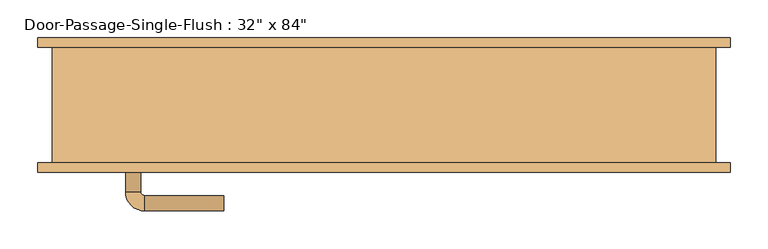
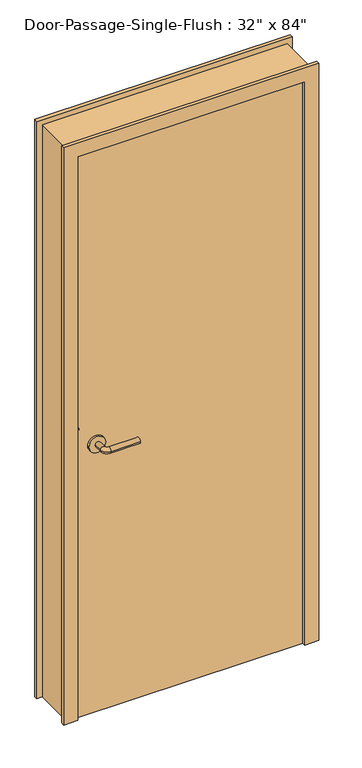
"""IFC4 building model written with IfcOpenShell, lengths in millimetres: door geometry."""

import ifcopenshell
import ifcopenshell.guid

model = None  # the IFC model being written
_history = None  # IfcOwnerHistory: only IFC2X3 demands one
_inside = {}  # id of a spatial element -> (the spatial element, [elements in it])
_under = {}  # id of a project, library or spatial element -> (it, [spatial elements below it])
_declared = {}  # id of a project -> (the project, [libraries it declares])
_typed = {}  # id of a type object -> (the type object, [elements of that type])
_made_of = {}  # id of a material, layer set ... -> (it, [elements and type objects made of it])


def new_model(schema):
    """Start an empty IFC model of exactly this schema.

    Asked for "IFC4X3", IfcOpenShell would pick the latest addendum, in which some entities
    have other attributes; the version numbers below select the first issue.
    IFC2X3 requires an IfcOwnerHistory on every rooted entity: one is made here for all.
    """
    global model, _history
    if schema == "IFC4X3":
        model = ifcopenshell.file(schema_version=(4, 3, 0, 0))
    else:
        model = ifcopenshell.file(schema=schema)
    _inside.clear()
    _under.clear()
    _declared.clear()
    _typed.clear()
    _made_of.clear()
    _history = None
    if model.schema == "IFC2X3":
        org = make("IfcOrganization", Name="unknown")
        user = make(
            "IfcPersonAndOrganization",
            ThePerson=make("IfcPerson", FamilyName="unknown"),
            TheOrganization=org,
        )
        app = make(
            "IfcApplication",
            ApplicationDeveloper=org,
            Version="unknown",
            ApplicationFullName="unknown",
            ApplicationIdentifier="unknown",
        )
        _history = make(
            "IfcOwnerHistory",
            OwningUser=user,
            OwningApplication=app,
            ChangeAction="ADDED",
            CreationDate=0,
        )
    return model


def make(cls, **values):
    """One entity of the class cls with the attributes given. An attribute that is None is left unset."""
    return model.create_entity(
        cls, **{name: value for name, value in values.items() if value is not None}
    )


def rooted(cls, **values):
    """An entity with a GlobalId (a new one), such as an element, a storey or a relation."""
    return make(cls, GlobalId=ifcopenshell.guid.new(), OwnerHistory=_history, **values)


def si_unit(unit_type, name, prefix=None):
    """IfcSIUnit, for example si_unit("LENGTHUNIT", "METRE", prefix="MILLI")."""
    return make("IfcSIUnit", UnitType=unit_type, Prefix=prefix, Name=name)


def assignment(units):
    """IfcUnitAssignment: the units of a project."""
    return None if units is None else make("IfcUnitAssignment", Units=units)


def point(xyz):
    """IfcCartesianPoint."""
    return None if xyz is None else make("IfcCartesianPoint", Coordinates=xyz)


def direction(xyz):
    """IfcDirection."""
    return None if xyz is None else make("IfcDirection", DirectionRatios=xyz)


def frame(location, z_axis=None, x_axis=None):
    """IfcAxis2Placement3D, a coordinate frame: its origin and axes. An axis left out is left unset."""
    return make(
        "IfcAxis2Placement3D",
        Location=point(location),
        Axis=direction(z_axis),
        RefDirection=direction(x_axis),
    )


def frame_2d(location, x_axis=None):
    """IfcAxis2Placement2D, a coordinate frame in the plane: its origin and x axis."""
    return make(
        "IfcAxis2Placement2D", Location=point(location), RefDirection=direction(x_axis)
    )


def origin():
    """The frame at (0, 0, 0) with its axes left unset."""
    return frame((0.0, 0.0, 0.0))


def origin_with_axes():
    """The frame at (0, 0, 0) with the z axis (0, 0, 1) and the x axis (1, 0, 0) written out."""
    return frame((0.0, 0.0, 0.0), z_axis=(0.0, 0.0, 1.0), x_axis=(1.0, 0.0, 0.0))


def place(relative_to, where):
    """IfcLocalPlacement: puts the frame where relative to a parent placement (None: the world)."""
    return make(
        "IfcLocalPlacement", PlacementRelTo=relative_to, RelativePlacement=where
    )


def context(
    kind, dimensions, precision=None, world=None, true_north=None, identifier=None
):
    """IfcGeometricRepresentationContext, for example the 3D "Model" context."""
    return make(
        "IfcGeometricRepresentationContext",
        ContextIdentifier=identifier,
        ContextType=kind,
        CoordinateSpaceDimension=dimensions,
        Precision=precision,
        WorldCoordinateSystem=world,
        TrueNorth=true_north,
    )


def project(units=None, contexts=None):
    """IfcProject with its units and contexts."""
    return rooted(
        "IfcProject",
        Name="project",
        RepresentationContexts=contexts,
        UnitsInContext=assignment(units),
    )


def spatial(cls, under=None, at=None, **own):
    """A site, building, storey or space (cls), placed at a placement, below another one or the project."""
    s = rooted(cls, ObjectPlacement=at, **own)
    if under is not None:
        _under.setdefault(under.id(), (under, []))[1].append(s)
    return s


def polyline(points):
    """IfcPolyline through the points."""
    return make("IfcPolyline", Points=[point(p) for p in points])


def circle_curve(where, radius):
    """IfcCircle in the frame where."""
    return make("IfcCircle", Position=where, Radius=radius)


def ellipse_curve(where, semi_axis1, semi_axis2):
    """IfcEllipse in the frame where."""
    return make(
        "IfcEllipse", Position=where, SemiAxis1=semi_axis1, SemiAxis2=semi_axis2
    )


def trimmed(basis, trim1, trim2, sense, master):
    """IfcTrimmedCurve: the piece of a basis curve between two trims."""
    return make(
        "IfcTrimmedCurve",
        BasisCurve=basis,
        Trim1=trim1,
        Trim2=trim2,
        SenseAgreement=sense,
        MasterRepresentation=master,
    )


def segment(curve, same_sense, transition):
    """IfcCompositeCurveSegment."""
    return make(
        "IfcCompositeCurveSegment",
        Transition=transition,
        SameSense=same_sense,
        ParentCurve=curve,
    )


def composite_curve(segments, self_intersect=None):
    """IfcCompositeCurve: segments joined end to end."""
    return make("IfcCompositeCurve", Segments=segments, SelfIntersect=self_intersect)


def outline(outer, holes=None, kind="AREA"):
    """IfcArbitraryClosedProfileDef: a profile drawn as a closed curve; with holes, ...WithVoids."""
    if holes is None:
        return make("IfcArbitraryClosedProfileDef", ProfileType=kind, OuterCurve=outer)
    return make(
        "IfcArbitraryProfileDefWithVoids",
        ProfileType=kind,
        OuterCurve=outer,
        InnerCurves=holes,
    )


def extrude(swept, where, along, depth):
    """IfcExtrudedAreaSolid: the profile swept, set in the frame where, extruded along a direction by depth."""
    return make(
        "IfcExtrudedAreaSolid",
        SweptArea=swept,
        Position=where,
        ExtrudedDirection=direction(along),
        Depth=depth,
    )


def faces_of(points, faces, orient=None, outer=None):
    """IfcFace entities. A face is a list of loops; a loop is a list of indices into points, from 0.

    orient and outer hold one flag for each loop. By default every Orientation is true, the
    first loop of a face is its IfcFaceOuterBound and the others are IfcFaceBound.
    """
    made = []
    for i, loops in enumerate(faces):
        bounds = []
        for j, loop in enumerate(loops):
            is_outer = j == 0 if outer is None else outer[i][j]
            bounds.append(
                make(
                    "IfcFaceOuterBound" if is_outer else "IfcFaceBound",
                    Bound=make("IfcPolyLoop", Polygon=[points[k] for k in loop]),
                    Orientation=True if orient is None else orient[i][j],
                )
            )
        made.append(make("IfcFace", Bounds=bounds))
    return made


def faceted_brep(points, faces, orient=None, outer=None, voids=None):
    """IfcFacetedBrep: a solid bounded by flat faces; with voids (closed shells), ...WithVoids."""
    shared = [point(p) for p in points]
    hull = make("IfcClosedShell", CfsFaces=faces_of(shared, faces, orient, outer))
    if voids is None:
        return make("IfcFacetedBrep", Outer=hull)
    return make(
        "IfcFacetedBrepWithVoids",
        Outer=hull,
        Voids=[
            make(cls, CfsFaces=faces_of(shared, fs, o, b)) for cls, fs, o, b in voids
        ],
    )


def shape(context_of_items, identifier, shape_type, items):
    """IfcShapeRepresentation: the items that make up one representation, for example the "Body"."""
    return make(
        "IfcShapeRepresentation",
        ContextOfItems=context_of_items,
        RepresentationIdentifier=identifier,
        RepresentationType=shape_type,
        Items=items,
    )


def source(mapping_origin, context_of_items, identifier, shape_type, items):
    """IfcRepresentationMap: a shape defined once, which mapped items show again and again."""
    return make(
        "IfcRepresentationMap",
        MappingOrigin=mapping_origin,
        MappedRepresentation=shape(context_of_items, identifier, shape_type, items),
    )


def transform(
    local_origin,
    x_axis=None,
    y_axis=None,
    z_axis=None,
    scale=None,
    scale2=None,
    scale3=None,
    uniform=True,
):
    """IfcCartesianTransformationOperator3D, or its non-uniform kind. x_axis, y_axis, z_axis: its Axis1, 2, 3."""
    if uniform:
        return make(
            "IfcCartesianTransformationOperator3D",
            Axis1=direction(x_axis),
            Axis2=direction(y_axis),
            LocalOrigin=point(local_origin),
            Scale=scale,
            Axis3=direction(z_axis),
        )
    return make(
        "IfcCartesianTransformationOperator3DnonUniform",
        Axis1=direction(x_axis),
        Axis2=direction(y_axis),
        LocalOrigin=point(local_origin),
        Scale=scale,
        Axis3=direction(z_axis),
        Scale2=scale2,
        Scale3=scale3,
    )


def mapped(mapping_source, mapping_target):
    """IfcMappedItem: shows the shape of a source again, moved by a transform."""
    return make(
        "IfcMappedItem", MappingSource=mapping_source, MappingTarget=mapping_target
    )


def made_of(thing, what):
    """Note that an element or type object is made of a material, layer set ...; save() writes the relation."""
    if what is not None:
        _made_of.setdefault(what.id(), (what, []))[1].append(thing)
    return thing


def element(
    cls,
    number,
    at=None,
    inside=None,
    cuts=None,
    type_object=None,
    material=None,
    context=None,
    identifier="Body",
    shape_type=None,
    held_by="IfcProductDefinitionShape",
    body=None,
    shapes=None,
    **own,
):
    """One element of the class cls, such as IfcWall. Its Tag is "e" and its number.

    at: its placement. inside: the storey or other place that contains it. cuts: it is an
    opening in that element (IfcRelVoidsElement). A single representation is given by context,
    identifier, shape_type and body (its items); several are given by shapes. held_by: the class
    of the entity that holds the representations. save() writes the other relations.
    """
    e = rooted(cls, Tag="e%d" % number, ObjectPlacement=at, **own)
    if body is not None:
        shapes = [shape(context, identifier, shape_type, body)]
    if shapes is not None:
        e.Representation = make(held_by, Representations=shapes)
    if inside is not None:
        _inside.setdefault(inside.id(), (inside, []))[1].append(e)
    if cuts is not None:
        rooted(
            "IfcRelVoidsElement", RelatingBuildingElement=cuts, RelatedOpeningElement=e
        )
    if type_object is not None:
        _typed.setdefault(type_object.id(), (type_object, []))[1].append(e)
    return made_of(e, material)


def aggregate(whole, parts):
    """IfcRelAggregates: a whole, such as a stair, and the parts it consists of."""
    return rooted("IfcRelAggregates", RelatingObject=whole, RelatedObjects=parts)


def save(model, path):
    """Write the relations noted so far, then the file.

    IfcRelAggregates (storeys below a building ...), IfcRelContainedInSpatialStructure (elements
    in a storey), IfcRelDefinesByType, IfcRelAssociatesMaterial and IfcRelDeclares: one each for
    every whole, place, type object, material and project.
    """
    for whole, parts in _under.values():
        aggregate(whole, parts)
    for where, things in _inside.values():
        rooted(
            "IfcRelContainedInSpatialStructure",
            RelatedElements=things,
            RelatingStructure=where,
        )
    for kind, things in _typed.values():
        rooted("IfcRelDefinesByType", RelatedObjects=things, RelatingType=kind)
    for what, things in _made_of.values():
        rooted("IfcRelAssociatesMaterial", RelatedObjects=things, RelatingMaterial=what)
    for by, libraries in _declared.values():
        rooted("IfcRelDeclares", RelatingContext=by, RelatedDefinitions=libraries)
    model.write(path)


def plane_surface(at):
    """IfcPlane: the flat surface through the origin of the frame at, square to its z axis."""
    return make("IfcPlane", Position=at)


def cylinder_surface(at, radius):
    """IfcCylindricalSurface: all points at the distance radius from the z axis of the frame at."""
    return make("IfcCylindricalSurface", Position=at, Radius=radius)


def revolved_surface(curve, axis_point, axis_direction):
    """IfcSurfaceOfRevolution: the curve turned about the line through axis_point along axis_direction."""
    return make(
        "IfcSurfaceOfRevolution",
        SweptCurve=make("IfcArbitraryOpenProfileDef", ProfileType="CURVE", Curve=curve),
        AxisPosition=make("IfcAxis1Placement", Location=point(axis_point), Axis=direction(axis_direction)),
    )


def advanced_brep(points, edges, surfaces, faces):
    """IfcAdvancedBrep: a solid bounded by faces that lie on surfaces and meet in shared edges.

    An edge is (start, end): straight between two places in points (the first is 0);
    or (start, end, curve); or (start, end, curve, False) where it runs against its curve.
    A face is (place in surfaces, loops), or (place, loops, False) where it looks against
    its surface's normal. A loop lists edges by number (the first is 1), with a minus sign
    where the edge is run from its end to its start. The first loop is the outer one.
    """
    corners = [point(p) for p in points]
    vertices = [make("IfcVertexPoint", VertexGeometry=c) for c in corners]
    made = []
    for start, end, *more in edges:
        made.append(
            make(
                "IfcEdgeCurve",
                EdgeStart=vertices[start],
                EdgeEnd=vertices[end],
                EdgeGeometry=more[0] if more else make("IfcPolyline", Points=[corners[start], corners[end]]),
                SameSense=more[1] if len(more) > 1 else True,
            )
        )
    hull = []
    for where, loops, *sense in faces:
        bounds = []
        for j, loop in enumerate(loops):
            ring = [make("IfcOrientedEdge", EdgeElement=made[abs(k) - 1], Orientation=k > 0) for k in loop]
            bounds.append(
                make(
                    "IfcFaceOuterBound" if j == 0 else "IfcFaceBound",
                    Bound=make("IfcEdgeLoop", EdgeList=ring),
                    Orientation=True,
                )
            )
        hull.append(make("IfcAdvancedFace", Bounds=bounds, FaceSurface=surfaces[where], SameSense=sense[0] if sense else True))
    return make("IfcAdvancedBrep", Outer=make("IfcClosedShell", CfsFaces=hull))


def door_3d684360(model_context):
    return source(origin(), model_context, "Body", "SolidModel", [
        advanced_brep(
        [(-341.390625, -23.75, 1016.0), (-321.390625, -23.75, 1016.0), (-341.390625, 6.25, 1016.0), (-321.390625, 6.25, 1016.0), (-316.390625, 11.25, 1016.0), (-316.390625, 31.25, 1016.0), (-211.390625, 31.25, 1016.0), (-211.390625, 11.25, 1016.0)],
        [
            (0, 1, circle_curve(frame((-331.390625, -23.75, 1016.0), z_axis=(0.0, -1.0, 0.0), x_axis=(1.0, 0.0, 0.0)), 10.0)),
            (1, 0, circle_curve(frame((-331.390625, -23.75, 1016.0), z_axis=(0.0, -1.0, 0.0), x_axis=(1.0, 0.0, 0.0)), 10.0)),
            (0, 2),
            (2, 3, circle_curve(frame((-331.390625, 6.25, 1016.0), z_axis=(0.0, -1.0, 0.0), x_axis=(1.0, 0.0, 0.0)), 10.0)),
            (3, 1),
            (3, 2, circle_curve(frame((-331.390625, 6.25, 1016.0), z_axis=(0.0, -1.0, 0.0), x_axis=(1.0, 0.0, 0.0)), 10.0)),
            (4, 3, circle_curve(frame((-316.390625, 6.25, 1016.0), z_axis=(0.0, 0.0, 1.0), x_axis=(-1.0, 0.0, 0.0)), 5.0)),
            (2, 5, circle_curve(frame((-316.390625, 6.25, 1016.0), z_axis=(0.0, 0.0, -1.0), x_axis=(-1.0, 0.0, 0.0)), 25.0)),
            (5, 4, circle_curve(frame((-316.390625, 21.25, 1016.0), z_axis=(-1.0, 0.0, 0.0), x_axis=(0.0, -1.0, 0.0)), 10.0)),
            (4, 5, circle_curve(frame((-316.390625, 21.25, 1016.0), z_axis=(-1.0, 0.0, 0.0), x_axis=(0.0, -1.0, 0.0)), 10.0)),
            (6, 7, circle_curve(frame((-211.390625, 21.25, 1016.0), z_axis=(1.0, 0.0, 0.0), x_axis=(0.0, -1.0, 0.0)), 10.0)),
            (7, 6, circle_curve(frame((-211.390625, 21.25, 1016.0), z_axis=(1.0, 0.0, 0.0), x_axis=(0.0, -1.0, 0.0)), 10.0)),
            (5, 6),
            (7, 4),
        ],
        [
            plane_surface(frame((-331.390625, -23.75, 1016.0), z_axis=(0.0, -1.0, 0.0), x_axis=(0.0, 0.0, 1.0))),
            cylinder_surface(frame((-331.390625, -23.75, 1016.0), z_axis=(0.0, -1.0, 0.0), x_axis=(1.0, 0.0, 0.0)), 10.0),
            revolved_surface(trimmed(ellipse_curve(frame((-331.390625, 6.25, 1016.0), z_axis=(0.0, -1.0, 0.0), x_axis=(1.0, 0.0, 0.0)), 10.0, 10.0), [point((-341.390625, 6.25, 1016.0))], [point((-321.390625, 6.25, 1016.0))], True, "CARTESIAN"), (-316.390625, 6.25, 1016.0), (0.0, 0.0, -1.0)),
            revolved_surface(trimmed(ellipse_curve(frame((-331.390625, 6.25, 1016.0), z_axis=(0.0, -1.0, 0.0), x_axis=(1.0, 0.0, 0.0)), 10.0, 10.0), [point((-321.390625, 6.25, 1016.0))], [point((-341.390625, 6.25, 1016.0))], True, "CARTESIAN"), (-316.390625, 6.25, 1016.0), (0.0, 0.0, -1.0)),
            plane_surface(frame((-211.390625, 21.25, 1016.0), z_axis=(1.0, 0.0, 0.0), x_axis=(0.0, 0.0, 1.0))),
            cylinder_surface(frame((-316.390625, 21.25, 1016.0), z_axis=(-1.0, 0.0, 0.0), x_axis=(0.0, -1.0, 0.0)), 10.0),
        ],
        [
            (0, [[1, 2]]),
            (1, [[-1, 3, 4, 5]]),
            (1, [[-2, -5, 6, -3]]),
            (2, [[7, -4, 8, 9]]),
            (3, [[-8, -6, -7, 10]]),
            (4, [[11, 12]]),
            (5, [[-9, 13, -12, 14]]),
            (5, [[-10, -14, -11, -13]]),
        ],
    ),
        extrude(outline(composite_curve([segment(trimmed(circle_curve(frame_2d((1016.0, -333.890625)), 30.0), [point((1016.0, -363.890625))], [point((1016.0, -303.890625))], False, "CARTESIAN"), True, "CONTINUOUS"), segment(trimmed(circle_curve(frame_2d((1016.0, -333.890625)), 30.0), [point((1016.0, -303.890625))], [point((1016.0, -363.890625))], False, "CARTESIAN"), True, "CONTINUOUS")], self_intersect=False)), frame((0.0, -31.75, 0.0), z_axis=(0.0, 1.0, 0.0), x_axis=(0.0, 0.0, 1.0)), (0.0, 0.0, 1.0), 8.0),
        advanced_brep(
        [(-341.390625, -90.55, 1016.0), (-321.390625, -90.55, 1016.0), (-321.390625, -120.55, 1016.0), (-341.390625, -120.55, 1016.0), (-316.390625, -125.55, 1016.0), (-316.390625, -145.55, 1016.0), (-211.390625, -145.55, 1016.0), (-211.390625, -125.55, 1016.0)],
        [
            (0, 1, circle_curve(frame((-331.390625, -90.55, 1016.0), z_axis=(0.0, 1.0, 0.0), x_axis=(1.0, 0.0, 0.0)), 10.0)),
            (1, 0, circle_curve(frame((-331.390625, -90.55, 1016.0), z_axis=(0.0, 1.0, 0.0), x_axis=(1.0, 0.0, 0.0)), 10.0)),
            (1, 2),
            (2, 3, circle_curve(frame((-331.390625, -120.55, 1016.0), z_axis=(0.0, 1.0, 0.0), x_axis=(1.0, 0.0, 0.0)), 10.0)),
            (3, 0),
            (3, 2, circle_curve(frame((-331.390625, -120.55, 1016.0), z_axis=(0.0, 1.0, 0.0), x_axis=(1.0, 0.0, 0.0)), 10.0)),
            (4, 5, circle_curve(frame((-316.390625, -135.55, 1016.0), z_axis=(-1.0, 0.0, 0.0), x_axis=(0.0, 1.0, 0.0)), 10.0)),
            (5, 3, circle_curve(frame((-316.390625, -120.55, 1016.0), z_axis=(0.0, 0.0, -1.0), x_axis=(-1.0, 0.0, 0.0)), 25.0)),
            (2, 4, circle_curve(frame((-316.390625, -120.55, 1016.0), z_axis=(0.0, 0.0, 1.0), x_axis=(-1.0, 0.0, 0.0)), 5.0)),
            (5, 4, circle_curve(frame((-316.390625, -135.55, 1016.0), z_axis=(-1.0, 0.0, 0.0), x_axis=(0.0, 1.0, 0.0)), 10.0)),
            (6, 7, circle_curve(frame((-211.390625, -135.55, 1016.0), z_axis=(1.0, 0.0, 0.0), x_axis=(0.0, 1.0, 0.0)), 10.0)),
            (7, 6, circle_curve(frame((-211.390625, -135.55, 1016.0), z_axis=(1.0, 0.0, 0.0), x_axis=(0.0, 1.0, 0.0)), 10.0)),
            (4, 7),
            (6, 5),
        ],
        [
            plane_surface(frame((-331.390625, -90.55, 1016.0), z_axis=(0.0, 1.0, 0.0), x_axis=(0.0, 0.0, 1.0))),
            cylinder_surface(frame((-331.390625, -90.55, 1016.0), z_axis=(0.0, 1.0, 0.0), x_axis=(1.0, 0.0, 0.0)), 10.0),
            revolved_surface(trimmed(ellipse_curve(frame((-331.390625, -120.55, 1016.0), z_axis=(0.0, -1.0, 0.0), x_axis=(1.0, 0.0, 0.0)), 10.0, 10.0), [point((-341.390625, -120.55, 1016.0))], [point((-321.390625, -120.55, 1016.0))], True, "CARTESIAN"), (-316.390625, -120.55, 1016.0), (0.0, 0.0, -1.0)),
            revolved_surface(trimmed(ellipse_curve(frame((-331.390625, -120.55, 1016.0), z_axis=(0.0, -1.0, 0.0), x_axis=(1.0, 0.0, 0.0)), 10.0, 10.0), [point((-321.390625, -120.55, 1016.0))], [point((-341.390625, -120.55, 1016.0))], True, "CARTESIAN"), (-316.390625, -120.55, 1016.0), (0.0, 0.0, -1.0)),
            plane_surface(frame((-211.390625, -135.55, 1016.0), z_axis=(1.0, 0.0, 0.0), x_axis=(0.0, 0.0, 1.0))),
            cylinder_surface(frame((-316.390625, -135.55, 1016.0), z_axis=(-1.0, 0.0, 0.0), x_axis=(0.0, 1.0, 0.0)), 10.0),
        ],
        [
            (0, [[1, 2]]),
            (1, [[3, 4, 5, -2]]),
            (1, [[-5, 6, -3, -1]]),
            (2, [[7, 8, -4, 9]]),
            (3, [[10, -9, -6, -8]]),
            (4, [[11, 12]]),
            (5, [[13, -11, 14, -7]]),
            (5, [[-14, -12, -13, -10]]),
        ],
    ),
        extrude(outline(composite_curve([segment(trimmed(circle_curve(frame_2d((1016.0, -333.890625)), 30.0), [point((1016.0, -363.890625))], [point((1016.0, -303.890625))], False, "CARTESIAN"), True, "CONTINUOUS"), segment(trimmed(circle_curve(frame_2d((1016.0, -333.890625)), 30.0), [point((1016.0, -303.890625))], [point((1016.0, -363.890625))], False, "CARTESIAN"), True, "CONTINUOUS")], self_intersect=False)), frame((0.0, -90.55, 0.0), z_axis=(0.0, 1.0, 0.0), x_axis=(0.0, 0.0, 1.0)), (0.0, 0.0, 1.0), 8.0),
        faceted_brep([(406.4, -95.25, 0.0), (406.4, -26.9875, 0.0), (390.525, -26.9875, 0.0), (390.525, 11.1125, 0.0), (406.4, 11.1125, 0.0), (406.4, 82.55, 0.0), (457.2, 82.55, 0.0), (457.2, 69.85, 0.0), (438.15, 69.85, 0.0), (438.15, -82.55, 0.0), (457.2, -82.55, 0.0), (457.2, -95.25, 0.0), (457.2, -95.25, 2184.4), (-457.2, -95.25, 2184.4), (-457.2, -95.25, 0.0), (-406.4, -95.25, 0.0), (-406.4, -95.25, 2133.6), (406.4, -95.25, 2133.6), (457.2, -82.55, 2184.4), (438.15, -82.55, 2165.35), (-438.15, -82.55, 2165.35), (-438.15, -82.55, 0.0), (-457.2, -82.55, 0.0), (-457.2, -82.55, 2184.4), (438.15, 69.85, 2165.35), (457.2, 69.85, 2184.4), (-457.2, 69.85, 2184.4), (-457.2, 69.85, 0.0), (-438.15, 69.85, 0.0), (-438.15, 69.85, 2165.35), (457.2, 82.55, 2184.4), (406.4, 82.55, 2133.6), (-406.4, 82.55, 2133.6), (-406.4, 82.55, 0.0), (-457.2, 82.55, 0.0), (-457.2, 82.55, 2184.4), (406.4, 11.1125, 2133.6), (390.525, 11.1125, 2117.725), (-390.525, 11.1125, 2117.725), (-390.525, 11.1125, 0.0), (-406.4, 11.1125, 0.0), (-406.4, 11.1125, 2133.6), (390.525, -26.9875, 2117.725), (406.4, -26.9875, 2133.6), (-406.4, -26.9875, 2133.6), (-406.4, -26.9875, 0.0), (-390.525, -26.9875, 0.0), (-390.525, -26.9875, 2117.725)], [[[0, 1, 2, 3, 4, 5, 6, 7, 8, 9, 10, 11]], [[11, 12, 13, 14, 15, 16, 17, 0]], [[10, 18, 12, 11]], [[9, 19, 20, 21, 22, 23, 18, 10]], [[8, 24, 19, 9]], [[7, 25, 26, 27, 28, 29, 24, 8]], [[6, 30, 25, 7]], [[5, 31, 32, 33, 34, 35, 30, 6]], [[4, 36, 31, 5]], [[3, 37, 38, 39, 40, 41, 36, 4]], [[2, 42, 37, 3]], [[1, 43, 44, 45, 46, 47, 42, 2]], [[0, 17, 43, 1]], [[18, 23, 13, 12]], [[24, 29, 20, 19]], [[30, 35, 26, 25]], [[36, 41, 32, 31]], [[42, 47, 38, 37]], [[17, 16, 44, 43]], [[15, 14, 22, 21, 28, 27, 34, 33, 40, 39, 46, 45]], [[23, 22, 14, 13]], [[29, 28, 21, 20]], [[35, 34, 27, 26]], [[41, 40, 33, 32]], [[47, 46, 39, 38]], [[16, 15, 45, 44]]]),
        extrude(outline(polyline([(406.4, -31.75), (406.4, -82.55), (-406.4, -82.55), (-406.4, -31.75), (406.4, -31.75)])), origin_with_axes(), (0.0, 0.0, 1.0), 2133.6),
    ])


if __name__ == "__main__":
    model = new_model("IFC4")
    model_context = context("Model", 3, world=origin())
    ifc_project = project(units=[si_unit("LENGTHUNIT", "METRE", prefix="MILLI")], contexts=[model_context])
    site = spatial("IfcSite", under=ifc_project)
    building = spatial("IfcBuilding", under=site)
    placement = place(None, origin())
    door_shape = door_3d684360(model_context)
    element("IfcDoor", 1, ObjectType="Door-Passage-Single-Flush : 32\" x 84\"", at=placement, inside=building, context=model_context, shape_type="MappedRepresentation", body=[
        mapped(door_shape, transform((0.0, 0.0, 0.0), x_axis=(1.0, 0.0, 0.0), y_axis=(0.0, 1.0, 0.0), z_axis=(0.0, 0.0, 1.0))),
    ])
    save(model, "model.ifc")

# Revit data of these elements
# Type "Door-Passage-Single-Flush : 32\" x 84\""
#   Type Mark = "10"
#   Assembly Code = "C1020"
#   Analytic Construction = "Wooden"
#   Thickness = 0' - 2"
#   Thermal Resistance (R) = 2.5876 (h·ft²·°F)/BTU
#   Swing Angle [instance default] = 90.00°
#   Strike Height = 3' - 4"
#   Rough Width [instance default] = 3' - 0"
#   Rough Height [instance default] = 7' - 4"
#   Masonry Inset [instance default] = 0' - 1"
#   Masonry Frame Depth = 0' - 5 3/4"
#   MF Opening Width [instance default] = 0' - 4"
#   MF Opening Height [instance default] = 0' - 4"
#   Inset Calculate [instance default] = 0' - 4"
#   Heat Transfer Coefficient (U) = 0.3865 BTU/(h·ft²·°F)
#   Height = 7' - 0"
#   Width = 2' - 8"
#   Masonry Frame [instance default] = yes
#   Dry Wall Frame [instance default] = no
#   Panel Material = Wood - Birch
#   Door Handle Material = Aluminum
#   Frame Material = Door - Frame
#   Visual Light Transmittance = 0
#   Solar Heat Gain Coefficient = 0
#   Function = (empty or 0)
#   Wall Closure = (empty or 0)
# Element 1 (IfcDoor, "Door-Passage-Single-Flush : 32\" x 84\"")
#   Rough Width = 2' - 10 1/2"
#   Rough Height = 7' - 1 1/4"
#   MF Opening Width = 0' - 2 1/2"
#   MF Opening Height = 0' - 1 1/4"
#   Inset Calculate = 0' - 3"
#   Masonry Frame = no
#   Dry Wall Frame = yes
#   Materials on its faces: "Door - Frame", "Aluminum", "Wood - Birch"
# Materials
#   "Wood - Birch": class "Unassigned", colour RGB 224 178 126, transparency 0
#   "Aluminum": class "Metal", colour RGB 244 244 244, transparency 0, Description = "Aluminum 6061", Cost = 0
#   "Door - Frame": class "Unassigned", colour RGB 118 70 51, transparency 0
